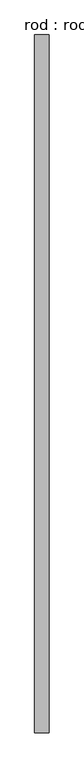
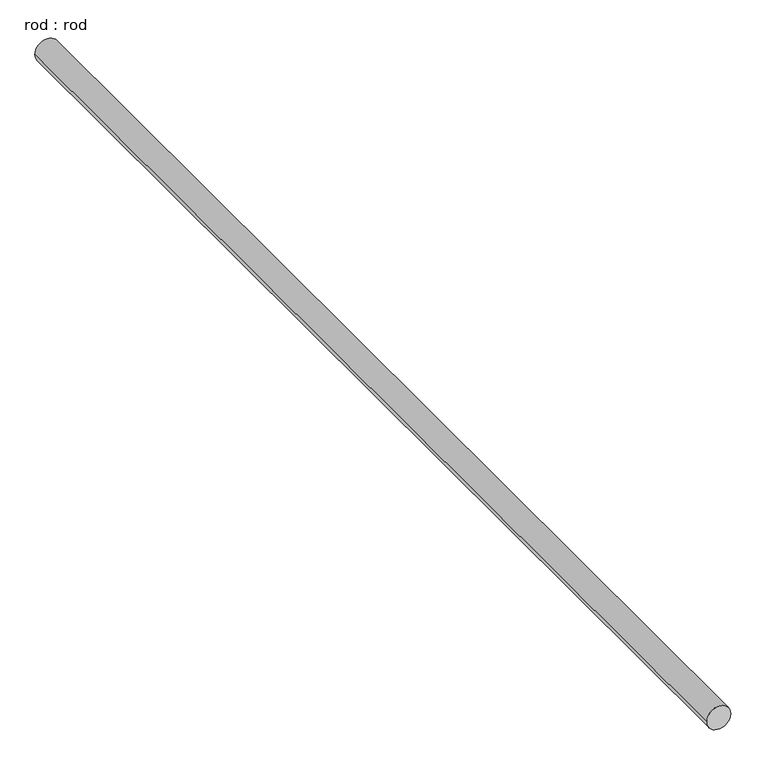
"""IFC4 building model written with IfcOpenShell, lengths in millimetres: proxy geometry, rod : rod."""

from ifc_helpers import new_model, si_unit, point, frame, frame_2d, origin, place, context, project, spatial, circle_curve, trimmed, segment, composite_curve, outline, extrude, source, transform, mapped, element, save


def rod_rod_af4d22da(model_context):
    return source(origin(), model_context, "Body", "SweptSolid", [
        extrude(outline(composite_curve([segment(trimmed(circle_curve(frame_2d((0.0108462, 0.0)), 200.0), [point((0.0108462, 200.0))], [point((0.0108462, -200.0))], False, "CARTESIAN"), True, "CONTINUOUS"), segment(trimmed(circle_curve(frame_2d((0.0108462, 0.0)), 200.0), [point((0.0108462, -200.0))], [point((0.0108462, 200.0))], False, "CARTESIAN"), True, "CONTINUOUS")], self_intersect=False)), frame((0.0, -5503.2718697, 0.0), z_axis=(0.0, 1.0, 0.0), x_axis=(0.0, 0.0, 1.0)), (0.0, 0.0, 1.0), 19192.0009701),
    ])


if __name__ == "__main__":
    model = new_model("IFC4")
    model_context = context("Model", 3, world=origin())
    ifc_project = project(units=[si_unit("LENGTHUNIT", "METRE", prefix="MILLI")], contexts=[model_context])
    site = spatial("IfcSite", under=ifc_project)
    building = spatial("IfcBuilding", under=site)
    placement = place(None, origin())
    rod_rod_shape = rod_rod_af4d22da(model_context)
    element("IfcBuildingElementProxy", 1, Name="rod : rod", ObjectType="rod : rod", at=placement, inside=building, context=model_context, shape_type="MappedRepresentation", body=[
        mapped(rod_rod_shape, transform((0.0, 0.0, 0.0), x_axis=(1.0, 0.0, 0.0), y_axis=(0.0, 1.0, 0.0), z_axis=(0.0, 0.0, 1.0))),
    ])
    save(model, "model.ifc")

# Revit data of these elements
# Type "rod : rod"
#   Default Elevation = 0
